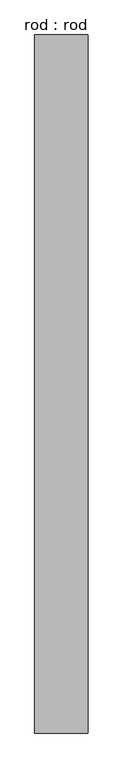
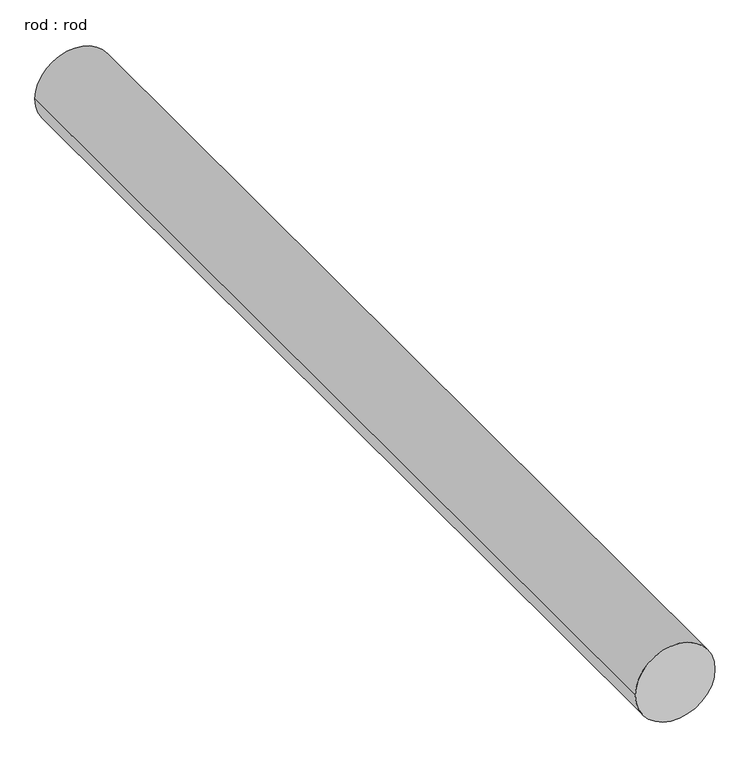
"""IFC4 building model written with IfcOpenShell, lengths in millimetres: proxy geometry, rod : rod."""

from ifc_helpers import new_model, si_unit, point, frame, frame_2d, origin, place, context, project, spatial, circle_curve, trimmed, segment, composite_curve, outline, extrude, source, transform, mapped, element, save


def rod_rod_61d853a1(model_context):
    return source(origin(), model_context, "Body", "SweptSolid", [
        extrude(outline(composite_curve([segment(trimmed(circle_curve(frame_2d((0.0108462, 0.0)), 200.0), [point((0.0108462, 200.0))], [point((0.0108462, -200.0))], False, "CARTESIAN"), True, "CONTINUOUS"), segment(trimmed(circle_curve(frame_2d((0.0108462, 0.0)), 200.0), [point((0.0108462, -200.0))], [point((0.0108462, 200.0))], False, "CARTESIAN"), True, "CONTINUOUS")], self_intersect=False)), frame((0.0, 1481.402324, 0.0), z_axis=(0.0, 1.0, 0.0), x_axis=(0.0, 0.0, 1.0)), (0.0, 0.0, 1.0), 5222.6525827),
    ])


if __name__ == "__main__":
    model = new_model("IFC4")
    model_context = context("Model", 3, world=origin())
    ifc_project = project(units=[si_unit("LENGTHUNIT", "METRE", prefix="MILLI")], contexts=[model_context])
    site = spatial("IfcSite", under=ifc_project)
    building = spatial("IfcBuilding", under=site)
    placement = place(None, origin())
    rod_rod_shape = rod_rod_61d853a1(model_context)
    element("IfcBuildingElementProxy", 1, Name="rod : rod", ObjectType="rod : rod", at=placement, inside=building, context=model_context, shape_type="MappedRepresentation", body=[
        mapped(rod_rod_shape, transform((0.0, 0.0, 0.0), x_axis=(1.0, 0.0, 0.0), y_axis=(0.0, 1.0, 0.0), z_axis=(0.0, 0.0, 1.0))),
    ])
    save(model, "model.ifc")

# Revit data of these elements
# Type "rod : rod"
#   Default Elevation = 0
